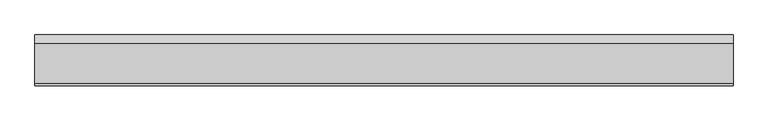
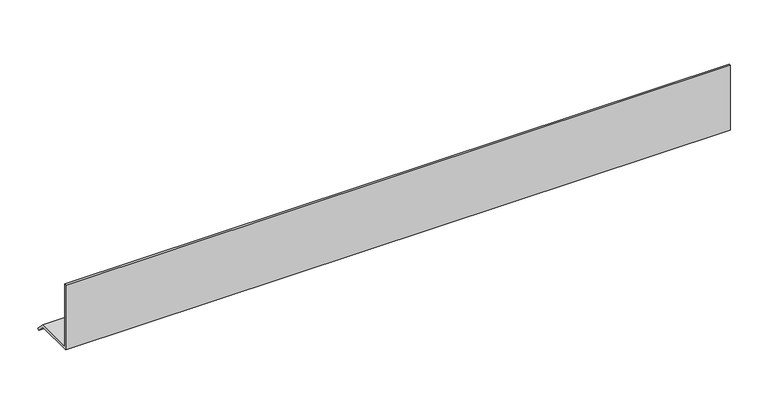
"""IFC4 building model written with IfcOpenShell, lengths in millimetres: proxy geometry, Generic Models 7:Generic Models 1:337419:Generic Models 1:337419 : Generic Models 7:Generic Models 1:337419:2 : Generic Models 7:Generic Models 1:337419:Generic Models 1:337419 : Generic Models 7:Generic Models 1:337419:301336."""

from ifc_helpers import new_model, si_unit, frame, origin, place, context, project, spatial, polyline, outline, extrude, source, transform, mapped, element, save


def generic_models_b8c2bb95(model_context):
    return source(origin(), model_context, "Body", "SweptSolid", [
        extrude(outline(polyline([(-536555.4753372, 2456.1595527), (-536555.4753372, 2560.5376777), (-536552.6972122, 2560.5376777), (-536552.6972122, 2458.9376777), (-536494.3964751, 2458.9376777), (-536481.6964751, 2446.2376777), (-536483.6609062, 2444.2732467), (-536495.5472122, 2456.1595527), (-536555.4753372, 2456.1595527)])), frame((592715.7367242, 0.0, 0.0), z_axis=(1.0, 0.0, 0.0), x_axis=(0.0, 1.0, 0.0)), (0.0, 0.0, 1.0), 1016.0),
    ])


if __name__ == "__main__":
    model = new_model("IFC4")
    model_context = context("Model", 3, world=origin())
    ifc_project = project(units=[si_unit("LENGTHUNIT", "METRE", prefix="MILLI")], contexts=[model_context])
    site = spatial("IfcSite", under=ifc_project)
    building = spatial("IfcBuilding", under=site)
    placement = place(None, origin())
    generic_models_shape = generic_models_b8c2bb95(model_context)
    element("IfcBuildingElementProxy", 1, Name="Generic Models 7:Generic Models 1:337419:Generic Models 1:337419 : Generic Models 7:Generic Models 1:337419:2 : Generic Models 7:Generic Models 1:337419:Generic Models 1:337419 : Generic Models 7:Generic Models 1:337419:301336", ObjectType="Generic Models 7:Generic Models 1:337419:Generic Models 1:337419 : Generic Models 7:Generic Models 1:337419:2 : Generic Models 7:Generic Models 1:337419:Generic Models 1:337419 : Generic Models 7:Generic Models 1:337419:301336", at=placement, inside=building, context=model_context, shape_type="MappedRepresentation", body=[
        mapped(generic_models_shape, transform((0.0, 0.0, 0.0), x_axis=(1.0, 0.0, 0.0), y_axis=(0.0, 1.0, 0.0), z_axis=(0.0, 0.0, 1.0))),
    ])
    save(model, "model.ifc")

# Revit data of these elements
# Type "Generic Models 7:Generic Models 1:337419:Generic Models 1:337419 : Generic Models 7:Generic Models 1:337419:2 : Generic Models 7:Generic Models 1:337419:Generic Models 1:337419 : Generic Models 7:Generic Models 1:337419:301336"
#   NameOverride = "Generic Models 7:Generic Models 1:337419:Generic Models 1:337419 : Generic Models 7:Generic Models 1:337419:301336"
#   ObjectTypeOverride = "Generic Models 1:337419 : Generic Models 7:Generic Models 1:337419"
#   Reference = "Generic Models 1"
#   Tag = "301336"
# Element 1 (IfcBuildingElementProxy, "Generic Models 7:Generic Models 1:337419:Generic Models 1:337419 : Generic Models 7:Generic Models 1:337419:2 : Generic Models 7:Generic Models 1:337419:Generic Models 1:337419 : Generic Models 7:Generic Models 1:337419:301336")
#   Materials on its faces: "BRAKE METAL FLASHING"
# Materials
#   "BRAKE METAL FLASHING": class "Unassigned", colour RGB 210 209 208, transparency 0, Cost = 0
